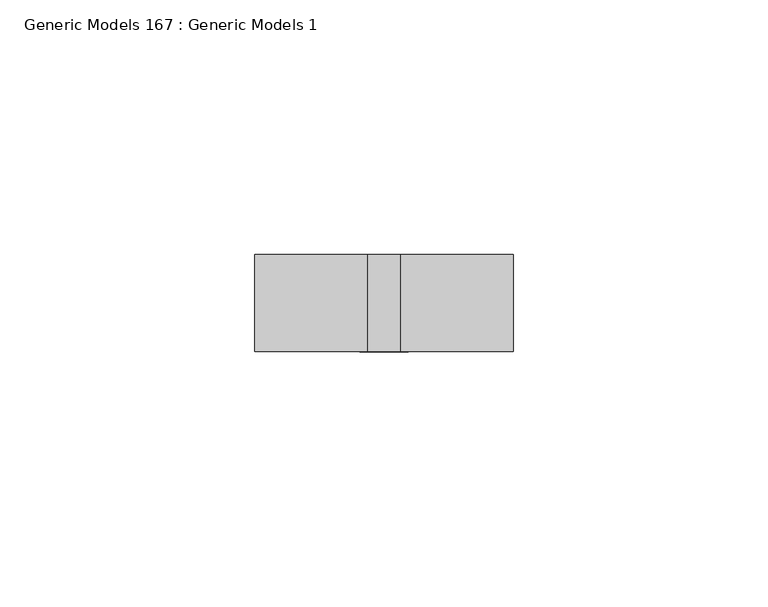
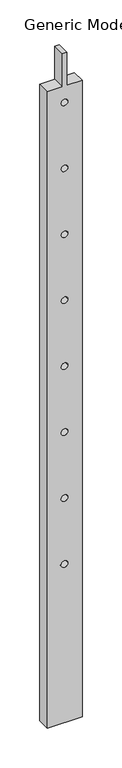
"""IFC4 building model written with IfcOpenShell, lengths in millimetres: proxy geometry, Generic Models 167 : Generic Models 1."""

from ifc_helpers import new_model, si_unit, point, frame, frame_2d, origin, place, context, project, spatial, polyline, circle_curve, trimmed, segment, composite_curve, outline, extrude, source, transform, mapped, element, save


def generic_models_167_generic_models_1_60d000e4(model_context):
    return source(origin(), model_context, "Body", "SweptSolid", [
        extrude(outline(polyline([(127777.621, -8229.7736296), (127777.621, -8251.9986296), (127828.421, -8251.9986296), (127828.421, -8258.3486296), (127777.621, -8258.3486296), (127777.621, -8280.5736296), (126796.546, -8280.5736296), (126796.546, -8229.7736296), (127777.621, -8229.7736296)]), holes=[composite_curve([segment(trimmed(circle_curve(frame_2d((127041.021, -8255.1736296)), 4.7625), [point((127041.021, -8259.9361296))], [point((127041.021, -8250.4111296))], True, "CARTESIAN"), True, "CONTINUOUS"), segment(trimmed(circle_curve(frame_2d((127041.021, -8255.1736296)), 4.7625), [point((127041.021, -8250.4111296))], [point((127041.021, -8259.9361296))], True, "CARTESIAN"), True, "CONTINUOUS")], self_intersect=False), composite_curve([segment(trimmed(circle_curve(frame_2d((127142.621, -8255.1736296)), 4.7625), [point((127142.621, -8259.9361296))], [point((127142.621, -8250.4111296))], True, "CARTESIAN"), True, "CONTINUOUS"), segment(trimmed(circle_curve(frame_2d((127142.621, -8255.1736296)), 4.7625), [point((127142.621, -8250.4111296))], [point((127142.621, -8259.9361296))], True, "CARTESIAN"), True, "CONTINUOUS")], self_intersect=False), composite_curve([segment(trimmed(circle_curve(frame_2d((127244.221, -8255.1736296)), 4.7625), [point((127244.221, -8259.9361296))], [point((127244.221, -8250.4111296))], True, "CARTESIAN"), True, "CONTINUOUS"), segment(trimmed(circle_curve(frame_2d((127244.221, -8255.1736296)), 4.7625), [point((127244.221, -8250.4111296))], [point((127244.221, -8259.9361296))], True, "CARTESIAN"), True, "CONTINUOUS")], self_intersect=False), composite_curve([segment(trimmed(circle_curve(frame_2d((127345.821, -8255.1736296)), 4.7625), [point((127345.821, -8259.9361296))], [point((127345.821, -8250.4111296))], True, "CARTESIAN"), True, "CONTINUOUS"), segment(trimmed(circle_curve(frame_2d((127345.821, -8255.1736296)), 4.7625), [point((127345.821, -8250.4111296))], [point((127345.821, -8259.9361296))], True, "CARTESIAN"), True, "CONTINUOUS")], self_intersect=False), composite_curve([segment(trimmed(circle_curve(frame_2d((127447.421, -8255.1736296)), 4.7625), [point((127447.421, -8259.9361296))], [point((127447.421, -8250.4111296))], True, "CARTESIAN"), True, "CONTINUOUS"), segment(trimmed(circle_curve(frame_2d((127447.421, -8255.1736296)), 4.7625), [point((127447.421, -8250.4111296))], [point((127447.421, -8259.9361296))], True, "CARTESIAN"), True, "CONTINUOUS")], self_intersect=False), composite_curve([segment(trimmed(circle_curve(frame_2d((127549.021, -8255.1736296)), 4.7625), [point((127549.021, -8259.9361296))], [point((127549.021, -8250.4111296))], True, "CARTESIAN"), True, "CONTINUOUS"), segment(trimmed(circle_curve(frame_2d((127549.021, -8255.1736296)), 4.7625), [point((127549.021, -8250.4111296))], [point((127549.021, -8259.9361296))], True, "CARTESIAN"), True, "CONTINUOUS")], self_intersect=False), composite_curve([segment(trimmed(circle_curve(frame_2d((127650.621, -8255.1736296)), 4.7625), [point((127650.621, -8259.9361296))], [point((127650.621, -8250.4111296))], True, "CARTESIAN"), True, "CONTINUOUS"), segment(trimmed(circle_curve(frame_2d((127650.621, -8255.1736296)), 4.7625), [point((127650.621, -8250.4111296))], [point((127650.621, -8259.9361296))], True, "CARTESIAN"), True, "CONTINUOUS")], self_intersect=False), composite_curve([segment(trimmed(circle_curve(frame_2d((127752.221, -8255.1736296)), 4.7625), [point((127752.221, -8259.9361296))], [point((127752.221, -8250.4111296))], True, "CARTESIAN"), True, "CONTINUOUS"), segment(trimmed(circle_curve(frame_2d((127752.221, -8255.1736296)), 4.7625), [point((127752.221, -8250.4111296))], [point((127752.221, -8259.9361296))], True, "CARTESIAN"), True, "CONTINUOUS")], self_intersect=False)]), frame((0.0, 542.6395048, 0.0), z_axis=(0.0, 1.0, 0.0), x_axis=(0.0, 0.0, 1.0)), (0.0, 0.0, 1.0), 19.05),
    ])


if __name__ == "__main__":
    model = new_model("IFC4")
    model_context = context("Model", 3, world=origin())
    ifc_project = project(units=[si_unit("LENGTHUNIT", "METRE", prefix="MILLI")], contexts=[model_context])
    site = spatial("IfcSite", under=ifc_project)
    building = spatial("IfcBuilding", under=site)
    placement = place(None, origin())
    generic_models_167_generic_models_1_shape = generic_models_167_generic_models_1_60d000e4(model_context)
    element("IfcBuildingElementProxy", 1, Name="Generic Models 167 : Generic Models 1", ObjectType="Generic Models 167 : Generic Models 1", at=placement, inside=building, context=model_context, shape_type="MappedRepresentation", body=[
        mapped(generic_models_167_generic_models_1_shape, transform((0.0, 0.0, 0.0), x_axis=(1.0, 0.0, 0.0), y_axis=(0.0, 1.0, 0.0), z_axis=(0.0, 0.0, 1.0))),
    ])
    save(model, "model.ifc")

# Revit data of these elements
# Element 1 (IfcBuildingElementProxy, "Generic Models 167 : Generic Models 1")
#   Materials on its faces: "_3/4\" x 1 1/2\" FLAT STOCK PAINTED STEEL POSTS"
# Materials
#   "_3/4\" x 1 1/2\" FLAT STOCK PAINTED STEEL POSTS": class "Generic", colour RGB 233 233 233, transparency 0, Cost = 0
